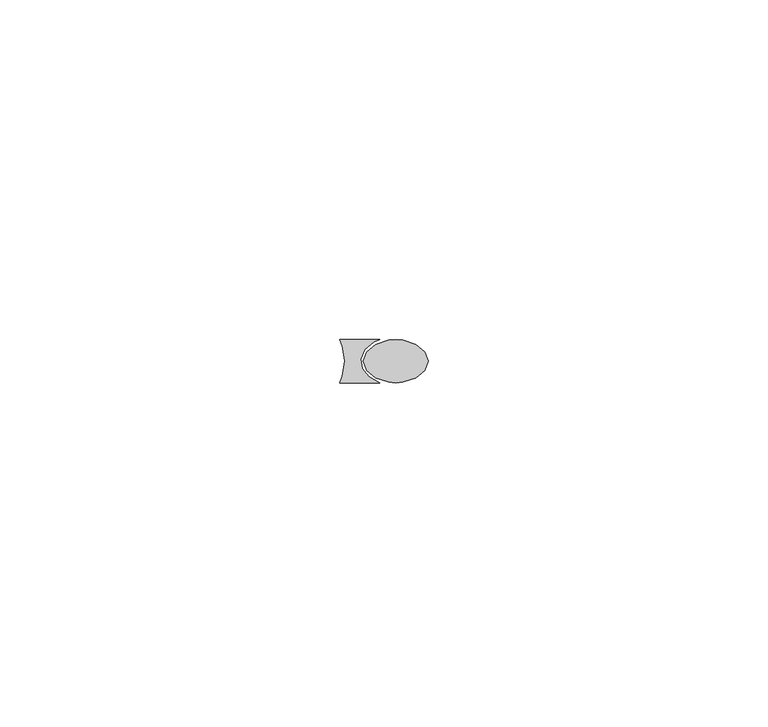
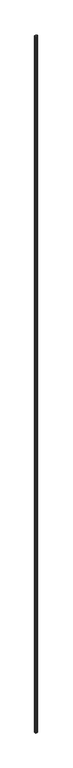
"""IFC4 building model written with IfcOpenShell, lengths in millimetres: proxy geometry, Generic Models 11:Generic Models 1:306267:Generic Models 1:306267 : Generic Models 11:Generic Models 1:306267:300405:Generic Models 1:306267:Generic Models 1:306267 : Generic Models 11:Generic Models 1:306267:300405 : Generic Models 11:Generic Models 1:306267:Generic Models 1:306267 : Generic Models 11:Generic Models 1:306267:300405:19 : Generic Models 11:Generic Models 1:306267:Generic Models 1:306267 : Generic Models 11:Generic Models 1:306267:300405:Generic Models 1:306267:Generic Models 1:306267 : Generic Models 11:Generic Models 1:306267:300405 : Generic Models 11:Generic Models 1:306267:Generic Models 1:306267 : Generic Models 11:Generic Models 1:306267:300405:300182."""

from ifc_helpers import new_model, si_unit, origin, origin_with_axes, place, context, project, spatial, polyline, outline, extrude, source, transform, mapped, element, save


def generic_models_92c7b32b(model_context):
    return source(origin(), model_context, "Body", "SweptSolid", [
        extrude(outline(polyline([(560274.3525794, -573568.5100798), (560275.6740734, -573567.4053457), (560277.5836877, -573566.7922646), (560278.6434436, -573566.7126607), (560279.7031996, -573566.7922646), (560281.6128138, -573567.4053457), (560282.9343079, -573568.5100798), (560283.4059436, -573569.8876607), (560282.9343079, -573571.2652416), (560281.6128138, -573572.3699756), (560279.7031996, -573572.9830568), (560278.6434436, -573573.0626607), (560277.5836877, -573572.9830568), (560275.6740734, -573572.3699756), (560274.3525794, -573571.2652416), (560273.8809436, -573569.8876607), (560274.3525794, -573568.5100798)])), origin_with_axes(), (0.0, 0.0, 1.0), 3695.7),
        extrude(outline(polyline([(560270.7891326, -573572.0968975), (560271.1028186, -573569.8876607), (560270.7891326, -573567.6784239), (560270.4117239, -573566.7126607), (560276.2798161, -573566.7126607), (560275.4195351, -573567.0989783), (560274.1099599, -573568.1824637), (560273.5096064, -573569.5327115), (560273.7123943, -573570.9384878), (560274.6865993, -573572.1798718), (560276.2798161, -573573.0626607), (560270.4117239, -573573.0626607), (560270.7891326, -573572.0968975)])), origin_with_axes(), (0.0, 0.0, 1.0), 3695.7),
    ])


if __name__ == "__main__":
    model = new_model("IFC4")
    model_context = context("Model", 3, world=origin())
    ifc_project = project(units=[si_unit("LENGTHUNIT", "METRE", prefix="MILLI")], contexts=[model_context])
    site = spatial("IfcSite", under=ifc_project)
    building = spatial("IfcBuilding", under=site)
    placement = place(None, origin())
    generic_models_shape = generic_models_92c7b32b(model_context)
    element("IfcBuildingElementProxy", 1, Name="Generic Models 11:Generic Models 1:306267:Generic Models 1:306267 : Generic Models 11:Generic Models 1:306267:300405:Generic Models 1:306267:Generic Models 1:306267 : Generic Models 11:Generic Models 1:306267:300405 : Generic Models 11:Generic Models 1:306267:Generic Models 1:306267 : Generic Models 11:Generic Models 1:306267:300405:19 : Generic Models 11:Generic Models 1:306267:Generic Models 1:306267 : Generic Models 11:Generic Models 1:306267:300405:Generic Models 1:306267:Generic Models 1:306267 : Generic Models 11:Generic Models 1:306267:300405 : Generic Models 11:Generic Models 1:306267:Generic Models 1:306267 : Generic Models 11:Generic Models 1:306267:300405:300182", ObjectType="Generic Models 11:Generic Models 1:306267:Generic Models 1:306267 : Generic Models 11:Generic Models 1:306267:300405:Generic Models 1:306267:Generic Models 1:306267 : Generic Models 11:Generic Models 1:306267:300405 : Generic Models 11:Generic Models 1:306267:Generic Models 1:306267 : Generic Models 11:Generic Models 1:306267:300405:19 : Generic Models 11:Generic Models 1:306267:Generic Models 1:306267 : Generic Models 11:Generic Models 1:306267:300405:Generic Models 1:306267:Generic Models 1:306267 : Generic Models 11:Generic Models 1:306267:300405 : Generic Models 11:Generic Models 1:306267:Generic Models 1:306267 : Generic Models 11:Generic Models 1:306267:300405:300182", at=placement, inside=building, context=model_context, shape_type="MappedRepresentation", body=[
        mapped(generic_models_shape, transform((0.0, 0.0, 0.0), x_axis=(1.0, 0.0, 0.0), y_axis=(0.0, 1.0, 0.0), z_axis=(0.0, 0.0, 1.0))),
    ])
    save(model, "model.ifc")

# Revit data of these elements
# Type "Generic Models 11:Generic Models 1:306267:Generic Models 1:306267 : Generic Models 11:Generic Models 1:306267:300405:Generic Models 1:306267:Generic Models 1:306267 : Generic Models 11:Generic Models 1:306267:300405 : Generic Models 11:Generic Models 1:306267:Generic Models 1:306267 : Generic Models 11:Generic Models 1:306267:300405:19 : Generic Models 11:Generic Models 1:306267:Generic Models 1:306267 : Generic Models 11:Generic Models 1:306267:300405:Generic Models 1:306267:Generic Models 1:306267 : Generic Models 11:Generic Models 1:306267:300405 : Generic Models 11:Generic Models 1:306267:Generic Models 1:306267 : Generic Models 11:Generic Models 1:306267:300405:300182"
#   NameOverride = "Generic Models 11:Generic Models 1:306267:Generic Models 1:306267 : Generic Models 11:Generic Models 1:306267:300405:Generic Models 1:306267:Generic Models 1:306267 : Generic Models 11:Generic Models 1:306267:300405 : Generic Models 11:Generic Models 1:306267:Generic Models 1:306267 : Generic Models 11:Generic Models 1:306267:300405:300182"
#   ObjectTypeOverride = "Generic Models 1:306267:Generic Models 1:306267 : Generic Models 11:Generic Models 1:306267:300405 : Generic Models 11:Generic Models 1:306267:Generic Models 1:306267 : Generic Models 11:Generic Models 1:306267:300405"
#   Reference = "Generic Models 1"
#   Tag = "300182"
# Element 1 (IfcBuildingElementProxy, "Generic Models 11:Generic Models 1:306267:Generic Models 1:306267 : Generic Models 11:Generic Models 1:306267:300405:Generic Models 1:306267:Generic Models 1:306267 : Generic Models 11:Generic Models 1:306267:300405 : Generic Models 11:Generic Models 1:306267:Generic Models 1:306267 : Generic Models 11:Generic Models 1:306267:300405:19 : Generic Models 11:Generic Models 1:306267:Generic Models 1:306267 : Generic Models 11:Generic Models 1:306267:300405:Generic Models 1:306267:Generic Models 1:306267 : Generic Models 11:Generic Models 1:306267:300405 : Generic Models 11:Generic Models 1:306267:Generic Models 1:306267 : Generic Models 11:Generic Models 1:306267:300405:300182")
#   Materials on its faces: "SEALANT & BACKER ROD, IF NECESSARY"
# Materials
#   "SEALANT & BACKER ROD, IF NECESSARY": class "Unassigned", colour RGB 120 120 120, transparency 0, Cost = 0
